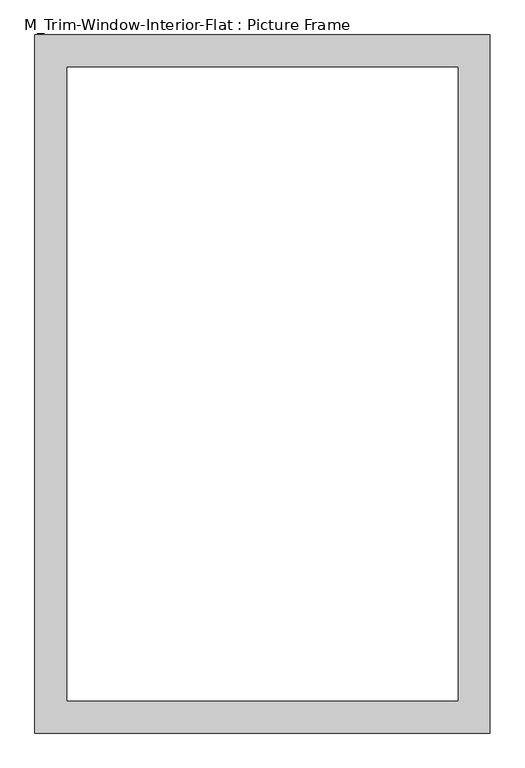
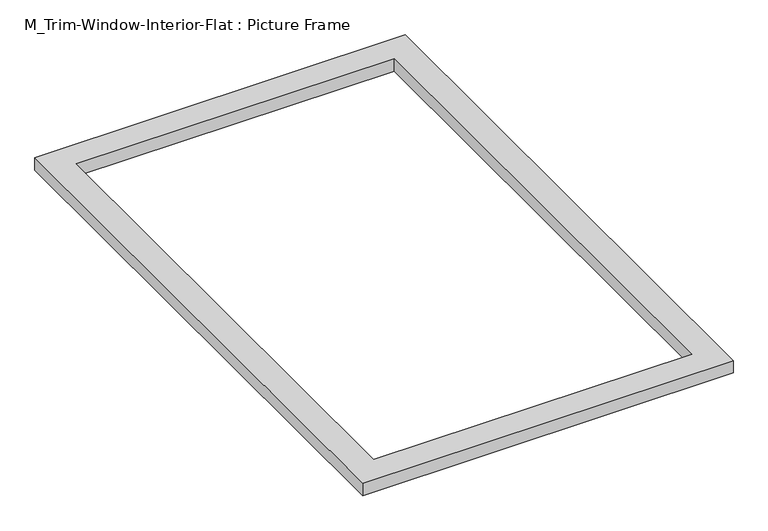
"""IFC4 building model written with IfcOpenShell, lengths in millimetres: proxy geometry, M_Trim-Window-Interior-Flat : Picture Frame."""

import ifcopenshell
import ifcopenshell.guid

model = None  # the IFC model being written
_history = None  # IfcOwnerHistory: only IFC2X3 demands one
_inside = {}  # id of a spatial element -> (the spatial element, [elements in it])
_under = {}  # id of a project, library or spatial element -> (it, [spatial elements below it])
_declared = {}  # id of a project -> (the project, [libraries it declares])
_typed = {}  # id of a type object -> (the type object, [elements of that type])
_made_of = {}  # id of a material, layer set ... -> (it, [elements and type objects made of it])


def new_model(schema):
    """Start an empty IFC model of exactly this schema.

    Asked for "IFC4X3", IfcOpenShell would pick the latest addendum, in which some entities
    have other attributes; the version numbers below select the first issue.
    IFC2X3 requires an IfcOwnerHistory on every rooted entity: one is made here for all.
    """
    global model, _history
    if schema == "IFC4X3":
        model = ifcopenshell.file(schema_version=(4, 3, 0, 0))
    else:
        model = ifcopenshell.file(schema=schema)
    _inside.clear()
    _under.clear()
    _declared.clear()
    _typed.clear()
    _made_of.clear()
    _history = None
    if model.schema == "IFC2X3":
        org = make("IfcOrganization", Name="unknown")
        user = make(
            "IfcPersonAndOrganization",
            ThePerson=make("IfcPerson", FamilyName="unknown"),
            TheOrganization=org,
        )
        app = make(
            "IfcApplication",
            ApplicationDeveloper=org,
            Version="unknown",
            ApplicationFullName="unknown",
            ApplicationIdentifier="unknown",
        )
        _history = make(
            "IfcOwnerHistory",
            OwningUser=user,
            OwningApplication=app,
            ChangeAction="ADDED",
            CreationDate=0,
        )
    return model


def make(cls, **values):
    """One entity of the class cls with the attributes given. An attribute that is None is left unset."""
    return model.create_entity(
        cls, **{name: value for name, value in values.items() if value is not None}
    )


def rooted(cls, **values):
    """An entity with a GlobalId (a new one), such as an element, a storey or a relation."""
    return make(cls, GlobalId=ifcopenshell.guid.new(), OwnerHistory=_history, **values)


def si_unit(unit_type, name, prefix=None):
    """IfcSIUnit, for example si_unit("LENGTHUNIT", "METRE", prefix="MILLI")."""
    return make("IfcSIUnit", UnitType=unit_type, Prefix=prefix, Name=name)


def assignment(units):
    """IfcUnitAssignment: the units of a project."""
    return None if units is None else make("IfcUnitAssignment", Units=units)


def point(xyz):
    """IfcCartesianPoint."""
    return None if xyz is None else make("IfcCartesianPoint", Coordinates=xyz)


def direction(xyz):
    """IfcDirection."""
    return None if xyz is None else make("IfcDirection", DirectionRatios=xyz)


def frame(location, z_axis=None, x_axis=None):
    """IfcAxis2Placement3D, a coordinate frame: its origin and axes. An axis left out is left unset."""
    return make(
        "IfcAxis2Placement3D",
        Location=point(location),
        Axis=direction(z_axis),
        RefDirection=direction(x_axis),
    )


def origin():
    """The frame at (0, 0, 0) with its axes left unset."""
    return frame((0.0, 0.0, 0.0))


def origin_with_axes():
    """The frame at (0, 0, 0) with the z axis (0, 0, 1) and the x axis (1, 0, 0) written out."""
    return frame((0.0, 0.0, 0.0), z_axis=(0.0, 0.0, 1.0), x_axis=(1.0, 0.0, 0.0))


def place(relative_to, where):
    """IfcLocalPlacement: puts the frame where relative to a parent placement (None: the world)."""
    return make(
        "IfcLocalPlacement", PlacementRelTo=relative_to, RelativePlacement=where
    )


def context(
    kind, dimensions, precision=None, world=None, true_north=None, identifier=None
):
    """IfcGeometricRepresentationContext, for example the 3D "Model" context."""
    return make(
        "IfcGeometricRepresentationContext",
        ContextIdentifier=identifier,
        ContextType=kind,
        CoordinateSpaceDimension=dimensions,
        Precision=precision,
        WorldCoordinateSystem=world,
        TrueNorth=true_north,
    )


def project(units=None, contexts=None):
    """IfcProject with its units and contexts."""
    return rooted(
        "IfcProject",
        Name="project",
        RepresentationContexts=contexts,
        UnitsInContext=assignment(units),
    )


def spatial(cls, under=None, at=None, **own):
    """A site, building, storey or space (cls), placed at a placement, below another one or the project."""
    s = rooted(cls, ObjectPlacement=at, **own)
    if under is not None:
        _under.setdefault(under.id(), (under, []))[1].append(s)
    return s


def polyline(points):
    """IfcPolyline through the points."""
    return make("IfcPolyline", Points=[point(p) for p in points])


def outline(outer, holes=None, kind="AREA"):
    """IfcArbitraryClosedProfileDef: a profile drawn as a closed curve; with holes, ...WithVoids."""
    if holes is None:
        return make("IfcArbitraryClosedProfileDef", ProfileType=kind, OuterCurve=outer)
    return make(
        "IfcArbitraryProfileDefWithVoids",
        ProfileType=kind,
        OuterCurve=outer,
        InnerCurves=holes,
    )


def extrude(swept, where, along, depth):
    """IfcExtrudedAreaSolid: the profile swept, set in the frame where, extruded along a direction by depth."""
    return make(
        "IfcExtrudedAreaSolid",
        SweptArea=swept,
        Position=where,
        ExtrudedDirection=direction(along),
        Depth=depth,
    )


def shape(context_of_items, identifier, shape_type, items):
    """IfcShapeRepresentation: the items that make up one representation, for example the "Body"."""
    return make(
        "IfcShapeRepresentation",
        ContextOfItems=context_of_items,
        RepresentationIdentifier=identifier,
        RepresentationType=shape_type,
        Items=items,
    )


def source(mapping_origin, context_of_items, identifier, shape_type, items):
    """IfcRepresentationMap: a shape defined once, which mapped items show again and again."""
    return make(
        "IfcRepresentationMap",
        MappingOrigin=mapping_origin,
        MappedRepresentation=shape(context_of_items, identifier, shape_type, items),
    )


def transform(
    local_origin,
    x_axis=None,
    y_axis=None,
    z_axis=None,
    scale=None,
    scale2=None,
    scale3=None,
    uniform=True,
):
    """IfcCartesianTransformationOperator3D, or its non-uniform kind. x_axis, y_axis, z_axis: its Axis1, 2, 3."""
    if uniform:
        return make(
            "IfcCartesianTransformationOperator3D",
            Axis1=direction(x_axis),
            Axis2=direction(y_axis),
            LocalOrigin=point(local_origin),
            Scale=scale,
            Axis3=direction(z_axis),
        )
    return make(
        "IfcCartesianTransformationOperator3DnonUniform",
        Axis1=direction(x_axis),
        Axis2=direction(y_axis),
        LocalOrigin=point(local_origin),
        Scale=scale,
        Axis3=direction(z_axis),
        Scale2=scale2,
        Scale3=scale3,
    )


def mapped(mapping_source, mapping_target):
    """IfcMappedItem: shows the shape of a source again, moved by a transform."""
    return make(
        "IfcMappedItem", MappingSource=mapping_source, MappingTarget=mapping_target
    )


def made_of(thing, what):
    """Note that an element or type object is made of a material, layer set ...; save() writes the relation."""
    if what is not None:
        _made_of.setdefault(what.id(), (what, []))[1].append(thing)
    return thing


def element(
    cls,
    number,
    at=None,
    inside=None,
    cuts=None,
    type_object=None,
    material=None,
    context=None,
    identifier="Body",
    shape_type=None,
    held_by="IfcProductDefinitionShape",
    body=None,
    shapes=None,
    **own,
):
    """One element of the class cls, such as IfcWall. Its Tag is "e" and its number.

    at: its placement. inside: the storey or other place that contains it. cuts: it is an
    opening in that element (IfcRelVoidsElement). A single representation is given by context,
    identifier, shape_type and body (its items); several are given by shapes. held_by: the class
    of the entity that holds the representations. save() writes the other relations.
    """
    e = rooted(cls, Tag="e%d" % number, ObjectPlacement=at, **own)
    if body is not None:
        shapes = [shape(context, identifier, shape_type, body)]
    if shapes is not None:
        e.Representation = make(held_by, Representations=shapes)
    if inside is not None:
        _inside.setdefault(inside.id(), (inside, []))[1].append(e)
    if cuts is not None:
        rooted(
            "IfcRelVoidsElement", RelatingBuildingElement=cuts, RelatedOpeningElement=e
        )
    if type_object is not None:
        _typed.setdefault(type_object.id(), (type_object, []))[1].append(e)
    return made_of(e, material)


def aggregate(whole, parts):
    """IfcRelAggregates: a whole, such as a stair, and the parts it consists of."""
    return rooted("IfcRelAggregates", RelatingObject=whole, RelatedObjects=parts)


def save(model, path):
    """Write the relations noted so far, then the file.

    IfcRelAggregates (storeys below a building ...), IfcRelContainedInSpatialStructure (elements
    in a storey), IfcRelDefinesByType, IfcRelAssociatesMaterial and IfcRelDeclares: one each for
    every whole, place, type object, material and project.
    """
    for whole, parts in _under.values():
        aggregate(whole, parts)
    for where, things in _inside.values():
        rooted(
            "IfcRelContainedInSpatialStructure",
            RelatedElements=things,
            RelatingStructure=where,
        )
    for kind, things in _typed.values():
        rooted("IfcRelDefinesByType", RelatedObjects=things, RelatingType=kind)
    for what, things in _made_of.values():
        rooted("IfcRelAssociatesMaterial", RelatedObjects=things, RelatingMaterial=what)
    for by, libraries in _declared.values():
        rooted("IfcRelDeclares", RelatingContext=by, RelatedDefinitions=libraries)
    model.write(path)


def m_trim_window_interior_flat_picture_frame_31bd2320(model_context):
    return source(origin(), model_context, "Body", "SweptSolid", [
        extrude(outline(polyline([(422.3, 47.3), (422.3, -1247.3), (-422.3, -1247.3), (-422.3, 47.3), (422.3, 47.3)]), holes=[polyline([(362.3, -12.7), (-362.3, -12.7), (-362.3, -1187.3), (362.3, -1187.3), (362.3, -12.7)])]), origin_with_axes(), (0.0, 0.0, 1.0), 30.0),
    ])


if __name__ == "__main__":
    model = new_model("IFC4")
    model_context = context("Model", 3, world=origin())
    ifc_project = project(units=[si_unit("LENGTHUNIT", "METRE", prefix="MILLI")], contexts=[model_context])
    site = spatial("IfcSite", under=ifc_project)
    building = spatial("IfcBuilding", under=site)
    placement = place(None, origin())
    m_trim_window_interior_flat_picture_frame_shape = m_trim_window_interior_flat_picture_frame_31bd2320(model_context)
    element("IfcBuildingElementProxy", 1, Name="M_Trim-Window-Interior-Flat : Picture Frame", ObjectType="M_Trim-Window-Interior-Flat : Picture Frame", at=placement, inside=building, context=model_context, shape_type="MappedRepresentation", body=[
        mapped(m_trim_window_interior_flat_picture_frame_shape, transform((0.0, 0.0, 0.0), x_axis=(1.0, 0.0, 0.0), y_axis=(0.0, 1.0, 0.0), z_axis=(0.0, 0.0, 1.0))),
    ])
    save(model, "model.ifc")

# Revit data of these elements
# Type "M_Trim-Window-Interior-Flat : Picture Frame"
#   Trim Thickness_Picture Frame = 30 mm
#   Trim Width = 60 mm
#   Trim Thickness_with Sill = 20 mm
#   Sill Thickness = 30 mm
#   Opening Width [instance default] = 600 mm
#   Opening Height [instance default] = 900 mm
#   Default Elevation = 1200 mm
#   Sill = no
#   Picture Frame = yes
#   Trim Material [instance default] = none
# Element 1 (IfcBuildingElementProxy, "M_Trim-Window-Interior-Flat : Picture Frame")
#   Opening Width = 750 mm
#   Opening Height = 1200 mm
#   Trim Material = Wood - Stained
#   Materials on its faces: "Wood - Stained"
# Materials
#   "Wood - Stained": class "Wood", colour RGB 227 170 128, transparency 0, Cost = 0
